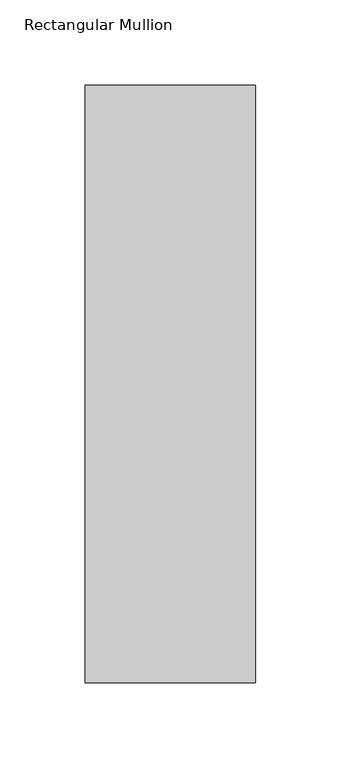
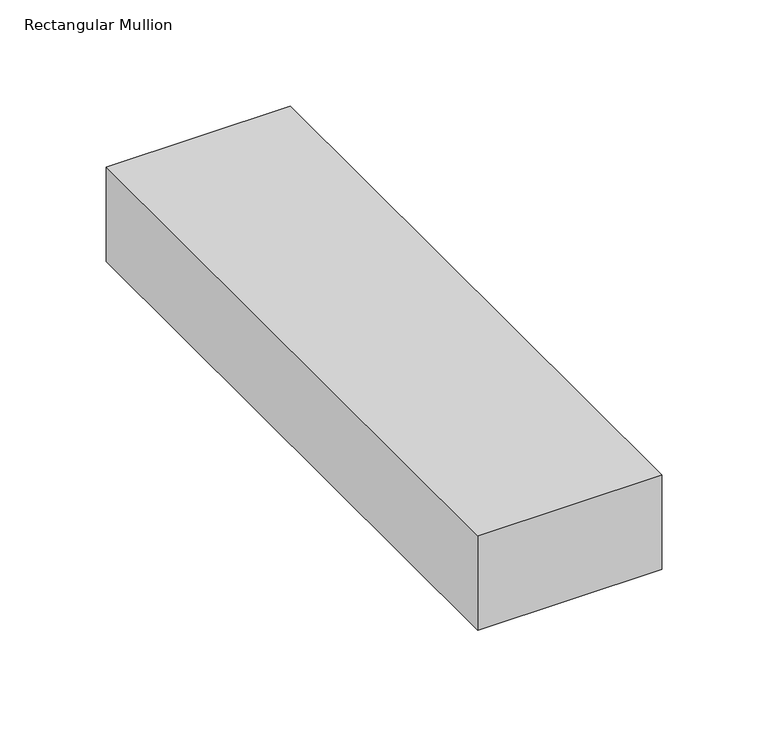
"""IFC4 building model written with IfcOpenShell, lengths in millimetres: member geometry, Rectangular Mullion : WWm-100x350-100mmOffset."""

from ifc_helpers import new_model, si_unit, frame, origin, place, context, project, spatial, polyline, outline, extrude, source, transform, mapped, element, save


def rectangular_mullion_fb2f718e(model_context):
    return source(origin(), model_context, "Body", "SweptSolid", [
        extrude(outline(polyline([(0.0, 175.0), (0.0, -175.0), (-100.0, -175.0), (-100.0, 175.0), (0.0, 175.0)])), frame((0.0, 0.0, -54.3459289), z_axis=(0.0, 0.0, 1.0), x_axis=(1.0, 0.0, 0.0)), (0.0, 0.0, 1.0), 54.3459289),
    ])


if __name__ == "__main__":
    model = new_model("IFC4")
    model_context = context("Model", 3, world=origin())
    ifc_project = project(units=[si_unit("LENGTHUNIT", "METRE", prefix="MILLI")], contexts=[model_context])
    site = spatial("IfcSite", under=ifc_project)
    building = spatial("IfcBuilding", under=site)
    placement = place(None, origin())
    rectangular_mullion_shape = rectangular_mullion_fb2f718e(model_context)
    element("IfcMember", 1, ObjectType="Rectangular Mullion : WWm-100x350-100mmOffset", at=placement, inside=building, context=model_context, shape_type="MappedRepresentation", body=[
        mapped(rectangular_mullion_shape, transform((0.0, 0.0, 0.0), x_axis=(1.0, 0.0, 0.0), y_axis=(0.0, 1.0, 0.0), z_axis=(0.0, 0.0, 1.0))),
    ])
    save(model, "model.ifc")

# Revit data of these elements
# Type "Rectangular Mullion : WWm-100x350-100mmOffset"
#   built-in parameter 1007304 = 1.14829 (stored number, unit not read)
#   built-in parameter 1007301 = 0.164042 (stored number, unit not read)
#   built-in parameter 1007300 = 0.164042 (stored number, unit not read)
# Element 1 (IfcMember, "Rectangular Mullion : WWm-100x350-100mmOffset")
#   Materials on its faces: "WW-EC-RGB-Mullion"
# Materials
#   "WW-EC-RGB-Mullion": class "Generic", colour RGB 255 255 255, transparency 0, Comments = "If region requests black mullions, switch asset color to RGB 25-25-25", Description = "Generic Color", Cost = 0
